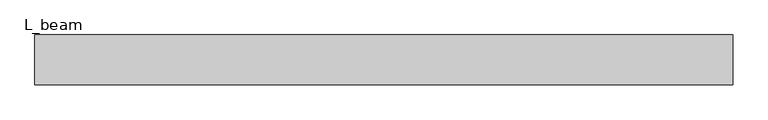
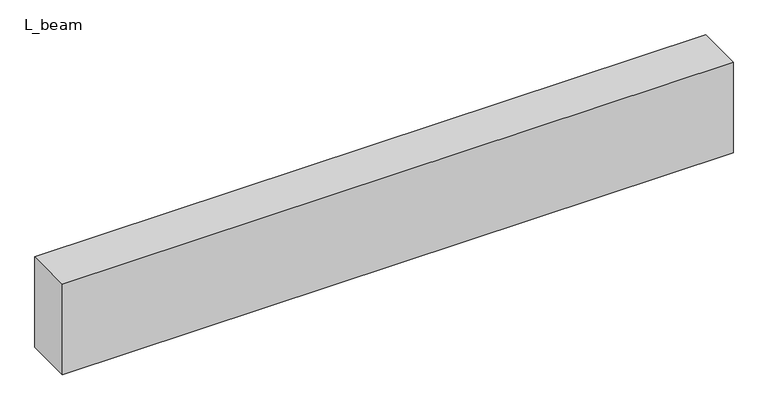
"""IFC4 building model written with IfcOpenShell, lengths in millimetres: beam geometry, 混凝土 - 矩形梁 : L_beam."""

from ifc_helpers import new_model, si_unit, frame, origin, place, context, project, spatial, polyline, outline, extrude, source, transform, mapped, element, save


def l_beam_e1ec5e6c(model_context):
    return source(origin(), model_context, "Body", "SweptSolid", [
        extrude(outline(polyline([(2105.0, 150.0), (2105.0, -150.0), (-2105.0, -150.0), (-2105.0, 150.0), (2105.0, 150.0)])), frame((0.0, 0.0, -300.0), z_axis=(0.0, 0.0, 1.0), x_axis=(1.0, 0.0, 0.0)), (0.0, 0.0, 1.0), 600.0),
    ])


if __name__ == "__main__":
    model = new_model("IFC4")
    model_context = context("Model", 3, world=origin())
    ifc_project = project(units=[si_unit("LENGTHUNIT", "METRE", prefix="MILLI")], contexts=[model_context])
    site = spatial("IfcSite", under=ifc_project)
    building = spatial("IfcBuilding", under=site)
    placement = place(None, origin())
    l_beam_shape = l_beam_e1ec5e6c(model_context)
    element("IfcBeam", 1, ObjectType="混凝土 - 矩形梁 : L_beam", at=placement, inside=building, context=model_context, shape_type="MappedRepresentation", body=[
        mapped(l_beam_shape, transform((0.0, 0.0, 0.0), x_axis=(1.0, 0.0, 0.0), y_axis=(0.0, 1.0, 0.0), z_axis=(0.0, 0.0, 1.0))),
    ])
    save(model, "model.ifc")

# Revit data of these elements
# Type "混凝土 - 矩形梁 : L_beam"
#   Length [instance default] = 1524 mm
#   b = 300 mm
#   h = 600 mm
#   Structural Material [instance default] = none
#   Assembly Code = ""
